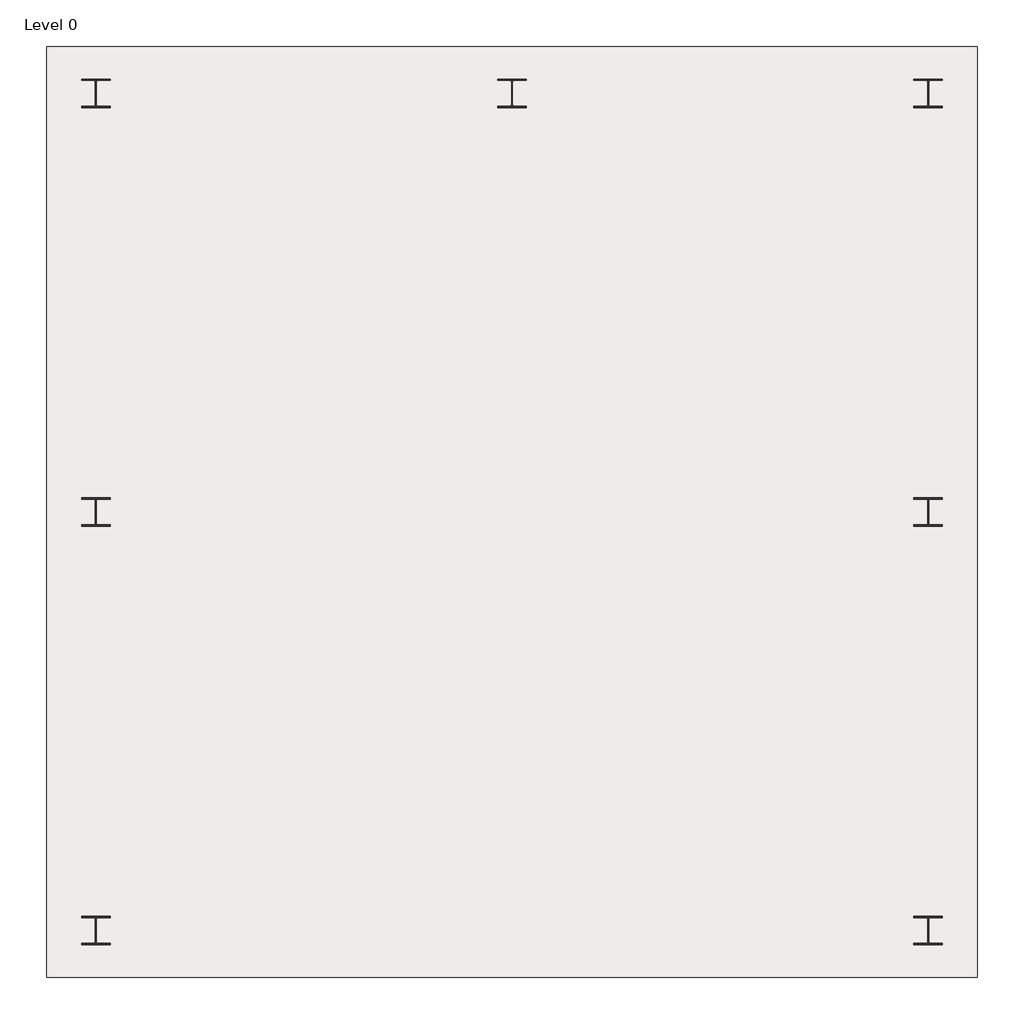
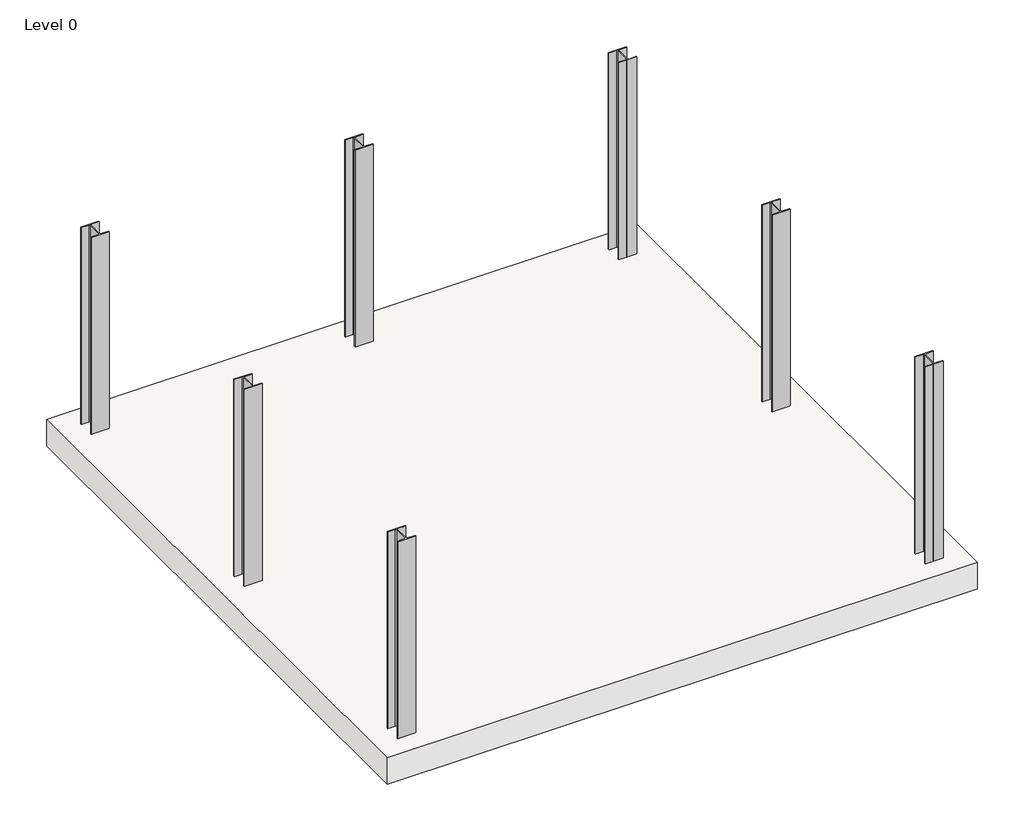
# One storey: 7 columns, 1 slab.
"""IFC4 building model written with IfcOpenShell, lengths in millimetres."""

import ifcopenshell
import ifcopenshell.guid

model = None  # the IFC model being written
_history = None  # IfcOwnerHistory: only IFC2X3 demands one
_inside = {}  # id of a spatial element -> (the spatial element, [elements in it])
_under = {}  # id of a project, library or spatial element -> (it, [spatial elements below it])
_declared = {}  # id of a project -> (the project, [libraries it declares])
_typed = {}  # id of a type object -> (the type object, [elements of that type])
_made_of = {}  # id of a material, layer set ... -> (it, [elements and type objects made of it])


def new_model(schema):
    """Start an empty IFC model of exactly this schema.

    Asked for "IFC4X3", IfcOpenShell would pick the latest addendum, in which some entities
    have other attributes; the version numbers below select the first issue.
    IFC2X3 requires an IfcOwnerHistory on every rooted entity: one is made here for all.
    """
    global model, _history
    if schema == "IFC4X3":
        model = ifcopenshell.file(schema_version=(4, 3, 0, 0))
    else:
        model = ifcopenshell.file(schema=schema)
    _inside.clear()
    _under.clear()
    _declared.clear()
    _typed.clear()
    _made_of.clear()
    _history = None
    if model.schema == "IFC2X3":
        org = make("IfcOrganization", Name="unknown")
        user = make(
            "IfcPersonAndOrganization",
            ThePerson=make("IfcPerson", FamilyName="unknown"),
            TheOrganization=org,
        )
        app = make(
            "IfcApplication",
            ApplicationDeveloper=org,
            Version="unknown",
            ApplicationFullName="unknown",
            ApplicationIdentifier="unknown",
        )
        _history = make(
            "IfcOwnerHistory",
            OwningUser=user,
            OwningApplication=app,
            ChangeAction="ADDED",
            CreationDate=0,
        )
    return model


def make(cls, **values):
    """One entity of the class cls with the attributes given. An attribute that is None is left unset."""
    return model.create_entity(
        cls, **{name: value for name, value in values.items() if value is not None}
    )


def rooted(cls, **values):
    """An entity with a GlobalId (a new one), such as an element, a storey or a relation."""
    return make(cls, GlobalId=ifcopenshell.guid.new(), OwnerHistory=_history, **values)


def si_unit(unit_type, name, prefix=None):
    """IfcSIUnit, for example si_unit("LENGTHUNIT", "METRE", prefix="MILLI")."""
    return make("IfcSIUnit", UnitType=unit_type, Prefix=prefix, Name=name)


def assignment(units):
    """IfcUnitAssignment: the units of a project."""
    return None if units is None else make("IfcUnitAssignment", Units=units)


def point(xyz):
    """IfcCartesianPoint."""
    return None if xyz is None else make("IfcCartesianPoint", Coordinates=xyz)


def direction(xyz):
    """IfcDirection."""
    return None if xyz is None else make("IfcDirection", DirectionRatios=xyz)


def frame(location, z_axis=None, x_axis=None):
    """IfcAxis2Placement3D, a coordinate frame: its origin and axes. An axis left out is left unset."""
    return make(
        "IfcAxis2Placement3D",
        Location=point(location),
        Axis=direction(z_axis),
        RefDirection=direction(x_axis),
    )


def frame_2d(location, x_axis=None):
    """IfcAxis2Placement2D, a coordinate frame in the plane: its origin and x axis."""
    return make(
        "IfcAxis2Placement2D", Location=point(location), RefDirection=direction(x_axis)
    )


def origin():
    """The frame at (0, 0, 0) with its axes left unset."""
    return frame((0.0, 0.0, 0.0))


def origin_with_axes():
    """The frame at (0, 0, 0) with the z axis (0, 0, 1) and the x axis (1, 0, 0) written out."""
    return frame((0.0, 0.0, 0.0), z_axis=(0.0, 0.0, 1.0), x_axis=(1.0, 0.0, 0.0))


def place(relative_to, where):
    """IfcLocalPlacement: puts the frame where relative to a parent placement (None: the world)."""
    return make(
        "IfcLocalPlacement", PlacementRelTo=relative_to, RelativePlacement=where
    )


def context(
    kind, dimensions, precision=None, world=None, true_north=None, identifier=None
):
    """IfcGeometricRepresentationContext, for example the 3D "Model" context."""
    return make(
        "IfcGeometricRepresentationContext",
        ContextIdentifier=identifier,
        ContextType=kind,
        CoordinateSpaceDimension=dimensions,
        Precision=precision,
        WorldCoordinateSystem=world,
        TrueNorth=true_north,
    )


def project(units=None, contexts=None):
    """IfcProject with its units and contexts."""
    return rooted(
        "IfcProject",
        Name="project",
        RepresentationContexts=contexts,
        UnitsInContext=assignment(units),
    )


def spatial(cls, under=None, at=None, **own):
    """A site, building, storey or space (cls), placed at a placement, below another one or the project."""
    s = rooted(cls, ObjectPlacement=at, **own)
    if under is not None:
        _under.setdefault(under.id(), (under, []))[1].append(s)
    return s


def polyline(points):
    """IfcPolyline through the points."""
    return make("IfcPolyline", Points=[point(p) for p in points])


def circle_curve(where, radius):
    """IfcCircle in the frame where."""
    return make("IfcCircle", Position=where, Radius=radius)


def trimmed(basis, trim1, trim2, sense, master):
    """IfcTrimmedCurve: the piece of a basis curve between two trims."""
    return make(
        "IfcTrimmedCurve",
        BasisCurve=basis,
        Trim1=trim1,
        Trim2=trim2,
        SenseAgreement=sense,
        MasterRepresentation=master,
    )


def segment(curve, same_sense, transition):
    """IfcCompositeCurveSegment."""
    return make(
        "IfcCompositeCurveSegment",
        Transition=transition,
        SameSense=same_sense,
        ParentCurve=curve,
    )


def composite_curve(segments, self_intersect=None):
    """IfcCompositeCurve: segments joined end to end."""
    return make("IfcCompositeCurve", Segments=segments, SelfIntersect=self_intersect)


def outline(outer, holes=None, kind="AREA"):
    """IfcArbitraryClosedProfileDef: a profile drawn as a closed curve; with holes, ...WithVoids."""
    if holes is None:
        return make("IfcArbitraryClosedProfileDef", ProfileType=kind, OuterCurve=outer)
    return make(
        "IfcArbitraryProfileDefWithVoids",
        ProfileType=kind,
        OuterCurve=outer,
        InnerCurves=holes,
    )


def extrude(swept, where, along, depth):
    """IfcExtrudedAreaSolid: the profile swept, set in the frame where, extruded along a direction by depth."""
    return make(
        "IfcExtrudedAreaSolid",
        SweptArea=swept,
        Position=where,
        ExtrudedDirection=direction(along),
        Depth=depth,
    )


def shape(context_of_items, identifier, shape_type, items):
    """IfcShapeRepresentation: the items that make up one representation, for example the "Body"."""
    return make(
        "IfcShapeRepresentation",
        ContextOfItems=context_of_items,
        RepresentationIdentifier=identifier,
        RepresentationType=shape_type,
        Items=items,
    )


def source(mapping_origin, context_of_items, identifier, shape_type, items):
    """IfcRepresentationMap: a shape defined once, which mapped items show again and again."""
    return make(
        "IfcRepresentationMap",
        MappingOrigin=mapping_origin,
        MappedRepresentation=shape(context_of_items, identifier, shape_type, items),
    )


def transform(
    local_origin,
    x_axis=None,
    y_axis=None,
    z_axis=None,
    scale=None,
    scale2=None,
    scale3=None,
    uniform=True,
):
    """IfcCartesianTransformationOperator3D, or its non-uniform kind. x_axis, y_axis, z_axis: its Axis1, 2, 3."""
    if uniform:
        return make(
            "IfcCartesianTransformationOperator3D",
            Axis1=direction(x_axis),
            Axis2=direction(y_axis),
            LocalOrigin=point(local_origin),
            Scale=scale,
            Axis3=direction(z_axis),
        )
    return make(
        "IfcCartesianTransformationOperator3DnonUniform",
        Axis1=direction(x_axis),
        Axis2=direction(y_axis),
        LocalOrigin=point(local_origin),
        Scale=scale,
        Axis3=direction(z_axis),
        Scale2=scale2,
        Scale3=scale3,
    )


def mapped(mapping_source, mapping_target):
    """IfcMappedItem: shows the shape of a source again, moved by a transform."""
    return make(
        "IfcMappedItem", MappingSource=mapping_source, MappingTarget=mapping_target
    )


def made_of(thing, what):
    """Note that an element or type object is made of a material, layer set ...; save() writes the relation."""
    if what is not None:
        _made_of.setdefault(what.id(), (what, []))[1].append(thing)
    return thing


def element(
    cls,
    number,
    at=None,
    inside=None,
    cuts=None,
    type_object=None,
    material=None,
    context=None,
    identifier="Body",
    shape_type=None,
    held_by="IfcProductDefinitionShape",
    body=None,
    shapes=None,
    **own,
):
    """One element of the class cls, such as IfcWall. Its Tag is "e" and its number.

    at: its placement. inside: the storey or other place that contains it. cuts: it is an
    opening in that element (IfcRelVoidsElement). A single representation is given by context,
    identifier, shape_type and body (its items); several are given by shapes. held_by: the class
    of the entity that holds the representations. save() writes the other relations.
    """
    e = rooted(cls, Tag="e%d" % number, ObjectPlacement=at, **own)
    if body is not None:
        shapes = [shape(context, identifier, shape_type, body)]
    if shapes is not None:
        e.Representation = make(held_by, Representations=shapes)
    if inside is not None:
        _inside.setdefault(inside.id(), (inside, []))[1].append(e)
    if cuts is not None:
        rooted(
            "IfcRelVoidsElement", RelatingBuildingElement=cuts, RelatedOpeningElement=e
        )
    if type_object is not None:
        _typed.setdefault(type_object.id(), (type_object, []))[1].append(e)
    return made_of(e, material)


def aggregate(whole, parts):
    """IfcRelAggregates: a whole, such as a stair, and the parts it consists of."""
    return rooted("IfcRelAggregates", RelatingObject=whole, RelatedObjects=parts)


def save(model, path):
    """Write the relations noted so far, then the file.

    IfcRelAggregates (storeys below a building ...), IfcRelContainedInSpatialStructure (elements
    in a storey), IfcRelDefinesByType, IfcRelAssociatesMaterial and IfcRelDeclares: one each for
    every whole, place, type object, material and project.
    """
    for whole, parts in _under.values():
        aggregate(whole, parts)
    for where, things in _inside.values():
        rooted(
            "IfcRelContainedInSpatialStructure",
            RelatedElements=things,
            RelatingStructure=where,
        )
    for kind, things in _typed.values():
        rooted("IfcRelDefinesByType", RelatedObjects=things, RelatingType=kind)
    for what, things in _made_of.values():
        rooted("IfcRelAssociatesMaterial", RelatedObjects=things, RelatingMaterial=what)
    for by, libraries in _declared.values():
        rooted("IfcRelDeclares", RelatingContext=by, RelatedDefinitions=libraries)
    model.write(path)


def uc_universal_columns_column_uc305x305x97_66ed23b3(model_context):
    return source(origin(), model_context, "Body", "SweptSolid", [
        extrude(outline(composite_curve([segment(polyline([(152.65, 153.95), (152.65, 138.55), (20.15, 138.55)]), True, "CONTINUOUS"), segment(trimmed(circle_curve(frame_2d((20.15, 123.35)), 15.2), [point((20.15, 138.55))], [point((4.95, 123.35))], True, "CARTESIAN"), True, "CONTINUOUS"), segment(polyline([(4.95, 123.35), (4.95, -123.35)]), True, "CONTINUOUS"), segment(trimmed(circle_curve(frame_2d((20.15, -123.35)), 15.2), [point((4.95, -123.35))], [point((20.15, -138.55))], True, "CARTESIAN"), True, "CONTINUOUS"), segment(polyline([(20.15, -138.55), (152.65, -138.55), (152.65, -153.95), (-152.65, -153.95), (-152.65, -138.55), (-20.15, -138.55)]), True, "CONTINUOUS"), segment(trimmed(circle_curve(frame_2d((-20.15, -123.35)), 15.2), [point((-20.15, -138.55))], [point((-4.95, -123.35))], True, "CARTESIAN"), True, "CONTINUOUS"), segment(polyline([(-4.95, -123.35), (-4.95, 123.35)]), True, "CONTINUOUS"), segment(trimmed(circle_curve(frame_2d((-20.15, 123.35)), 15.2), [point((-4.95, 123.35))], [point((-20.15, 138.55))], True, "CARTESIAN"), True, "CONTINUOUS"), segment(polyline([(-20.15, 138.55), (-152.65, 138.55), (-152.65, 153.95), (152.65, 153.95)]), True, "CONTINUOUS")], self_intersect=False)), origin_with_axes(), (0.0, 0.0, 1.0), 3530.0),
    ])


def uc_universal_columns_column_uc305x305x97_78c6f2b7(model_context):
    return source(origin(), model_context, "Body", "SweptSolid", [
        extrude(outline(composite_curve([segment(polyline([(152.65, -153.95), (-152.65, -153.95), (-152.65, -138.55), (-20.15, -138.55)]), True, "CONTINUOUS"), segment(trimmed(circle_curve(frame_2d((-20.15, -123.35)), 15.2), [point((-20.15, -138.55))], [point((-4.95, -123.35))], True, "CARTESIAN"), True, "CONTINUOUS"), segment(polyline([(-4.95, -123.35), (-4.95, 123.35)]), True, "CONTINUOUS"), segment(trimmed(circle_curve(frame_2d((-20.15, 123.35)), 15.2), [point((-4.95, 123.35))], [point((-20.15, 138.55))], True, "CARTESIAN"), True, "CONTINUOUS"), segment(polyline([(-20.15, 138.55), (-152.65, 138.55), (-152.65, 153.95), (152.65, 153.95), (152.65, 138.55), (20.15, 138.55)]), True, "CONTINUOUS"), segment(trimmed(circle_curve(frame_2d((20.15, 123.35)), 15.2), [point((20.15, 138.55))], [point((4.95, 123.35))], True, "CARTESIAN"), True, "CONTINUOUS"), segment(polyline([(4.95, 123.35), (4.95, -123.35)]), True, "CONTINUOUS"), segment(trimmed(circle_curve(frame_2d((20.15, -123.35)), 15.2), [point((4.95, -123.35))], [point((20.15, -138.55))], True, "CARTESIAN"), True, "CONTINUOUS"), segment(polyline([(20.15, -138.55), (152.65, -138.55), (152.65, -153.95)]), True, "CONTINUOUS")], self_intersect=False)), origin_with_axes(), (0.0, 0.0, 1.0), 3530.0),
    ])


model = new_model("IFC4")

# Units and contexts
model_context = context("Model", 3, world=origin())
ifc_project = project(units=[si_unit("LENGTHUNIT", "METRE", prefix="MILLI")], contexts=[model_context])

# Site, building, storey
site = spatial("IfcSite", under=ifc_project)
building = spatial("IfcBuilding", under=site)
storey = spatial("IfcBuildingStorey", under=building, Name="Level 0", Elevation=0.0)

# Columns
placement = place(None, origin())
uc_universal_columns_column_uc305x305x97_shape = uc_universal_columns_column_uc305x305x97_66ed23b3(model_context)
element("IfcColumn", 1, ObjectType="UC-Universal Columns-Column : UC305x305x97", at=placement, inside=storey, context=model_context, shape_type="MappedRepresentation", body=[
    mapped(uc_universal_columns_column_uc305x305x97_shape, transform((-4963.5138059, 4965.2875035, 0.0), x_axis=(1.0, 0.0, 0.0), y_axis=(0.0, 1.0, 0.0), z_axis=(0.0, 0.0, 1.0))),
])
element("IfcColumn", 2, ObjectType="UC-Universal Columns-Column : UC305x305x97", at=placement, inside=storey, context=model_context, shape_type="MappedRepresentation", body=[
    mapped(uc_universal_columns_column_uc305x305x97_shape, transform((3977.6728301, -4027.830418, 0.0), x_axis=(-1.0, 0.0, 0.0), y_axis=(0.0, -1.0, 0.0), z_axis=(0.0, 0.0, 1.0))),
])
element("IfcColumn", 3, ObjectType="UC-Universal Columns-Column : UC305x305x97", at=placement, inside=storey, context=model_context, shape_type="MappedRepresentation", body=[
    mapped(uc_universal_columns_column_uc305x305x97_shape, transform((-492.9204879, 4965.2875035, 0.0), x_axis=(1.0, 0.0, 0.0), y_axis=(0.0, 1.0, 0.0), z_axis=(0.0, 0.0, 1.0))),
])
element("IfcColumn", 4, ObjectType="UC-Universal Columns-Column : UC305x305x97", at=placement, inside=storey, context=model_context, shape_type="MappedRepresentation", body=[
    mapped(uc_universal_columns_column_uc305x305x97_shape, transform((3977.6728301, 468.7285428, 0.0), x_axis=(-1.0, 0.0, 0.0), y_axis=(0.0, -1.0, 0.0), z_axis=(0.0, 0.0, 1.0))),
])
uc_universal_columns_column_uc305x305x97_2_shape = uc_universal_columns_column_uc305x305x97_78c6f2b7(model_context)
element("IfcColumn", 5, ObjectType="UC-Universal Columns-Column : UC305x305x97", at=placement, inside=storey, context=model_context, shape_type="MappedRepresentation", body=[
    mapped(uc_universal_columns_column_uc305x305x97_2_shape, transform((-4963.5138059, -4027.830418, 0.0), x_axis=(1.0, 0.0, 0.0), y_axis=(0.0, 1.0, 0.0), z_axis=(0.0, 0.0, 1.0))),
])
element("IfcColumn", 6, ObjectType="UC-Universal Columns-Column : UC305x305x97", at=placement, inside=storey, context=model_context, shape_type="MappedRepresentation", body=[
    mapped(uc_universal_columns_column_uc305x305x97_2_shape, transform((3977.6728301, 4965.2875035, 0.0), x_axis=(-1.0, 0.0, 0.0), y_axis=(0.0, -1.0, 0.0), z_axis=(0.0, 0.0, 1.0))),
])
element("IfcColumn", 7, ObjectType="UC-Universal Columns-Column : UC305x305x97", at=placement, inside=storey, context=model_context, shape_type="MappedRepresentation", body=[
    mapped(uc_universal_columns_column_uc305x305x97_2_shape, transform((-4963.5138059, 468.7285428, 0.0), x_axis=(1.0, 0.0, 0.0), y_axis=(0.0, 1.0, 0.0), z_axis=(0.0, 0.0, 1.0))),
])

# Slab
element("IfcSlab", 8, ObjectType="Floor-Grnd-Susp_65Scr-80Ins-100Blk-75PC", at=placement, inside=storey, context=model_context, shape_type="SweptSolid", body=[
    extrude(outline(polyline([(4507.0795121, 5468.7285428), (4507.0795121, -4531.2714572), (-5492.9204879, -4531.2714572), (-5492.9204879, 5468.7285428), (4507.0795121, 5468.7285428)])), frame((0.0, 0.0, -470.0), z_axis=(0.0, 0.0, 1.0), x_axis=(1.0, 0.0, 0.0)), (0.0, 0.0, 1.0), 470.0),
])

save(model, "model.ifc")

# Revit data of these elements
# Project information
#   Project Issue Date = "Issue Date"
#   Project Status = "Project Status"
#   Client Name = "Owner"
#   Project Address = "Enter address here"
#   Project Name = "Project Name"
#   Project Number = "Project Number"
# Type "UC-Universal Columns-Column : UC305x305x97"
#   Section Name Key = "UC305x305x97"
#   Width = 30.53 cm
#   Web Thickness = 0.99 cm
#   Web Fillet = 1.52 cm
#   Warping Constant = 1560000.0 cm⁶
#   Torsional Moment of Inertia = 91.20 cm⁴
#   Section Area = 123.0 cm²
#   Plastic Modulus weak axis = 726.0 cm³
#   Plastic Modulus strong axis = 1592.0 cm³
#   Nominal Weight = 96.8996 kgf/m
#   Moment of Inertia weak axis = 7308.00 cm⁴
#   Moment of Inertia strong axis = 22249.00 cm⁴
#   Height = 30.79 cm
#   Flange Thickness = 1.54 cm
#   Elastic Modulus weak axis = 479.0 cm³
#   Elastic Modulus strong axis = 1445.0 cm³
#   Centroid Vertical = 15.395 cm
#   Centroid Horizontal = 15.265 cm
#   Bolt Spacing = 14.0 cm
#   Structural Material [instance default] = Metal - Steel 43-275
#   Type Comments = ""
#   Assembly Code = ""
# Type "Floor-Grnd-Susp_65Scr-80Ins-100Blk-75PC"
#   Keynote = "E60/130"
#   Function = 0
#   Layers, outside or top first: 0.065 m "Concrete, Sand/Cement Screed" (function 4); 0 m "Vapor Retarder" (function 100); 0.08 m "Rigid insulation" (function 3); 0.15 m "Air" (function 3); 0 m "Damp-proofing" (function 100); 0.1 m "Concrete Masonry, Floor Block" (function 1); 0.075 m "Concrete, Precast" (function 1)
# Elements 1, 2, 3, 4, 5, 6, 7 (IfcColumn, "UC-Universal Columns-Column : UC305x305x97")
#   Viktor_Change = no
#   Structural Material = Metal - Steel 43-275
#   Phase Created = New Construction
#   Materials on its faces: "Metal - Steel 43-275"
# Element 8 (IfcSlab, "Floor-Grnd-Susp_65Scr-80Ins-100Blk-75PC")
#   Height Offset From Level = 0 m
#   built-in parameter 1001954 = 1
#   Phase Created = New Construction
#   Materials on its faces: "Concrete, Precast", "Concrete, Sand/Cement Screed"
# Materials
#   "Metal - Steel 43-275": class "Metal", colour RGB 247 247 247, transparency 0, Cost = 0
#   "Concrete, Sand/Cement Screed": class "Concrete", colour RGB 127 127 127, transparency 0, Description = "Concrete slab topping", Cost = 0
#   "Vapor Retarder": class "Generic", colour RGB 120 120 120, transparency 0, Description = "Polyethylene film membrane", Cost = 0
#   "Rigid insulation": class "Generic", colour RGB 127 127 127, transparency 0, Description = "Rigid foam insulation board", Cost = 0
#   "Air": class "Gas", colour RGB 255 255 255, transparency 0, Description = "Air", Cost = 0
#   "Damp-proofing": class "Generic", colour RGB 127 127 127, transparency 0, Description = "Damp-proofing", Cost = 0
#   "Concrete Masonry, Floor Block": class "Concrete", colour RGB 181 181 181, transparency 0, Description = "physical material", Cost = 0
#   "Concrete, Precast": class "Concrete", colour RGB 192 192 192, transparency 0, Description = "Precast concrete", Cost = 0
